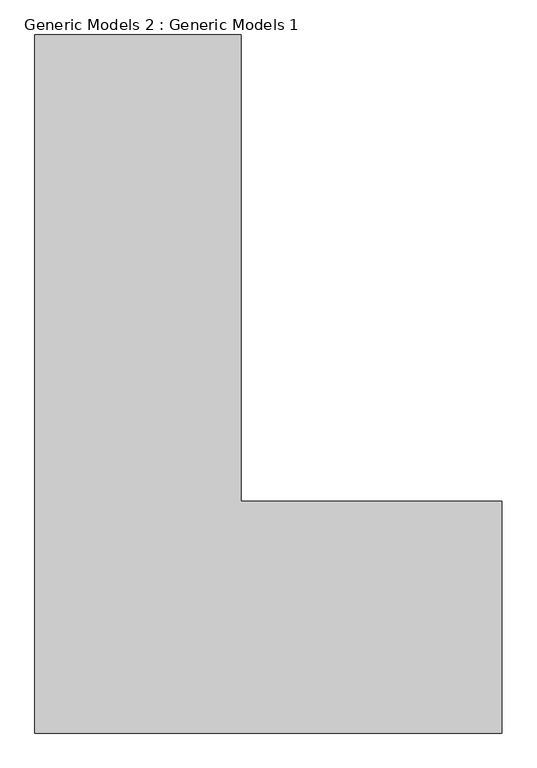
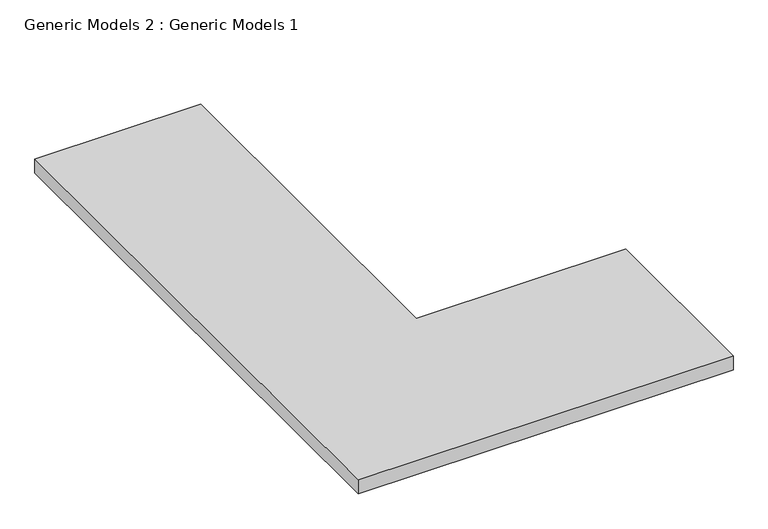
"""IFC4 building model written with IfcOpenShell, lengths in millimetres: furniture geometry, Generic Models 2 : Generic Models 1."""

from ifc_helpers import new_model, si_unit, frame, origin, place, context, project, spatial, polyline, outline, extrude, source, transform, mapped, element, save


def generic_models_2_generic_models_1_74315e81(model_context):
    return source(origin(), model_context, "Body", "SweptSolid", [
        extrude(outline(polyline([(28936.6402986, -12141.6330088), (29501.7902986, -12141.6330088), (29501.7902986, -13417.9830088), (30215.7652986, -13417.9830088), (30215.7652986, -14052.9830088), (28936.6402986, -14052.9830088), (28936.6402986, -12141.6330088)])), frame((0.0, 0.0, 4419.6), z_axis=(0.0, 0.0, 1.0), x_axis=(1.0, 0.0, 0.0)), (0.0, 0.0, 1.0), 50.8),
    ])


if __name__ == "__main__":
    model = new_model("IFC4")
    model_context = context("Model", 3, world=origin())
    ifc_project = project(units=[si_unit("LENGTHUNIT", "METRE", prefix="MILLI")], contexts=[model_context])
    site = spatial("IfcSite", under=ifc_project)
    building = spatial("IfcBuilding", under=site)
    placement = place(None, origin())
    generic_models_2_generic_models_1_shape = generic_models_2_generic_models_1_74315e81(model_context)
    element("IfcFurniture", 1, ObjectType="Generic Models 2 : Generic Models 1", at=placement, inside=building, context=model_context, shape_type="MappedRepresentation", body=[
        mapped(generic_models_2_generic_models_1_shape, transform((0.0, 0.0, 0.0), x_axis=(1.0, 0.0, 0.0), y_axis=(0.0, 1.0, 0.0), z_axis=(0.0, 0.0, 1.0))),
    ])
    save(model, "model.ifc")

# Revit data of these elements
# Element 1 (IfcFurniture, "Generic Models 2 : Generic Models 1")
#   Materials on its faces: "casework"
# Materials
#   "casework": class "Generic", colour RGB 209 209 209, transparency 0, Cost = 0
